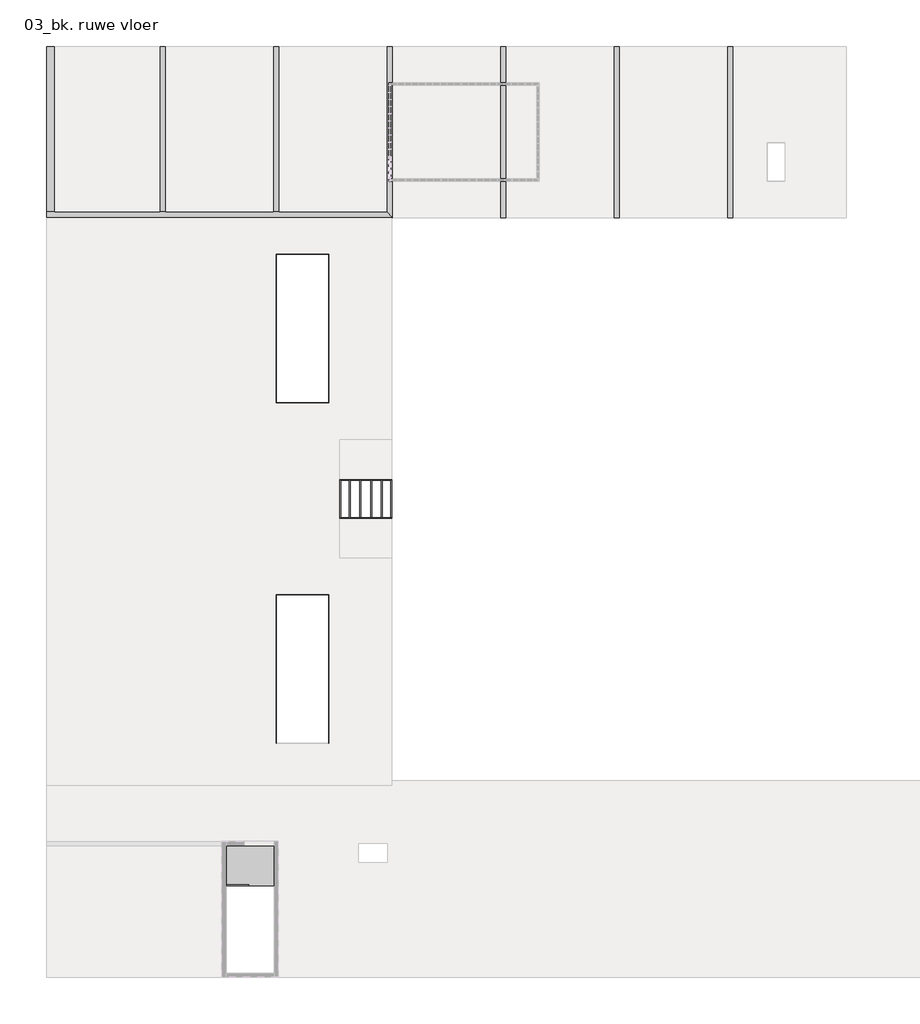
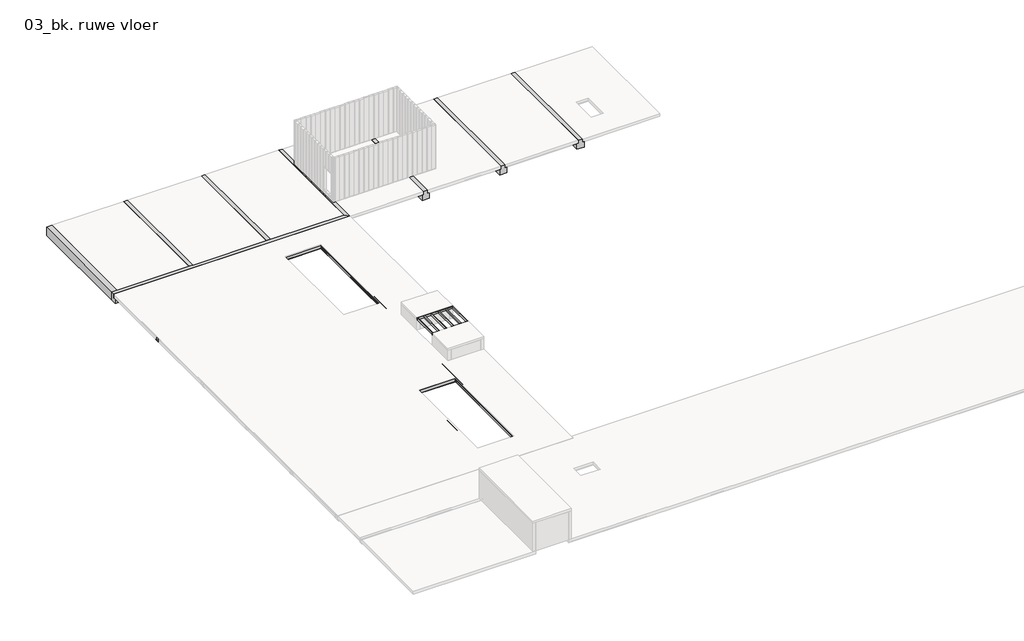
# One storey, part 9 of 9: 26 beams, 1 stair.
"""IFC4 building model written with IfcOpenShell, lengths in millimetres."""

import ifcopenshell
import ifcopenshell.guid

model = None  # the IFC model being written
_history = None  # IfcOwnerHistory: only IFC2X3 demands one
_inside = {}  # id of a spatial element -> (the spatial element, [elements in it])
_under = {}  # id of a project, library or spatial element -> (it, [spatial elements below it])
_declared = {}  # id of a project -> (the project, [libraries it declares])
_typed = {}  # id of a type object -> (the type object, [elements of that type])
_made_of = {}  # id of a material, layer set ... -> (it, [elements and type objects made of it])


def new_model(schema):
    """Start an empty IFC model of exactly this schema.

    Asked for "IFC4X3", IfcOpenShell would pick the latest addendum, in which some entities
    have other attributes; the version numbers below select the first issue.
    IFC2X3 requires an IfcOwnerHistory on every rooted entity: one is made here for all.
    """
    global model, _history
    if schema == "IFC4X3":
        model = ifcopenshell.file(schema_version=(4, 3, 0, 0))
    else:
        model = ifcopenshell.file(schema=schema)
    _inside.clear()
    _under.clear()
    _declared.clear()
    _typed.clear()
    _made_of.clear()
    _history = None
    if model.schema == "IFC2X3":
        org = make("IfcOrganization", Name="unknown")
        user = make(
            "IfcPersonAndOrganization",
            ThePerson=make("IfcPerson", FamilyName="unknown"),
            TheOrganization=org,
        )
        app = make(
            "IfcApplication",
            ApplicationDeveloper=org,
            Version="unknown",
            ApplicationFullName="unknown",
            ApplicationIdentifier="unknown",
        )
        _history = make(
            "IfcOwnerHistory",
            OwningUser=user,
            OwningApplication=app,
            ChangeAction="ADDED",
            CreationDate=0,
        )
    return model


def make(cls, **values):
    """One entity of the class cls with the attributes given. An attribute that is None is left unset."""
    return model.create_entity(
        cls, **{name: value for name, value in values.items() if value is not None}
    )


def rooted(cls, **values):
    """An entity with a GlobalId (a new one), such as an element, a storey or a relation."""
    return make(cls, GlobalId=ifcopenshell.guid.new(), OwnerHistory=_history, **values)


def si_unit(unit_type, name, prefix=None):
    """IfcSIUnit, for example si_unit("LENGTHUNIT", "METRE", prefix="MILLI")."""
    return make("IfcSIUnit", UnitType=unit_type, Prefix=prefix, Name=name)


def assignment(units):
    """IfcUnitAssignment: the units of a project."""
    return None if units is None else make("IfcUnitAssignment", Units=units)


def point(xyz):
    """IfcCartesianPoint."""
    return None if xyz is None else make("IfcCartesianPoint", Coordinates=xyz)


def direction(xyz):
    """IfcDirection."""
    return None if xyz is None else make("IfcDirection", DirectionRatios=xyz)


def frame(location, z_axis=None, x_axis=None):
    """IfcAxis2Placement3D, a coordinate frame: its origin and axes. An axis left out is left unset."""
    return make(
        "IfcAxis2Placement3D",
        Location=point(location),
        Axis=direction(z_axis),
        RefDirection=direction(x_axis),
    )


def frame_2d(location, x_axis=None):
    """IfcAxis2Placement2D, a coordinate frame in the plane: its origin and x axis."""
    return make(
        "IfcAxis2Placement2D", Location=point(location), RefDirection=direction(x_axis)
    )


def origin():
    """The frame at (0, 0, 0) with its axes left unset."""
    return frame((0.0, 0.0, 0.0))


def place(relative_to, where):
    """IfcLocalPlacement: puts the frame where relative to a parent placement (None: the world)."""
    return make(
        "IfcLocalPlacement", PlacementRelTo=relative_to, RelativePlacement=where
    )


def context(
    kind, dimensions, precision=None, world=None, true_north=None, identifier=None
):
    """IfcGeometricRepresentationContext, for example the 3D "Model" context."""
    return make(
        "IfcGeometricRepresentationContext",
        ContextIdentifier=identifier,
        ContextType=kind,
        CoordinateSpaceDimension=dimensions,
        Precision=precision,
        WorldCoordinateSystem=world,
        TrueNorth=true_north,
    )


def project(units=None, contexts=None):
    """IfcProject with its units and contexts."""
    return rooted(
        "IfcProject",
        Name="project",
        RepresentationContexts=contexts,
        UnitsInContext=assignment(units),
    )


def spatial(cls, under=None, at=None, **own):
    """A site, building, storey or space (cls), placed at a placement, below another one or the project."""
    s = rooted(cls, ObjectPlacement=at, **own)
    if under is not None:
        _under.setdefault(under.id(), (under, []))[1].append(s)
    return s


def polyline(points):
    """IfcPolyline through the points."""
    return make("IfcPolyline", Points=[point(p) for p in points])


def circle_curve(where, radius):
    """IfcCircle in the frame where."""
    return make("IfcCircle", Position=where, Radius=radius)


def trimmed(basis, trim1, trim2, sense, master):
    """IfcTrimmedCurve: the piece of a basis curve between two trims."""
    return make(
        "IfcTrimmedCurve",
        BasisCurve=basis,
        Trim1=trim1,
        Trim2=trim2,
        SenseAgreement=sense,
        MasterRepresentation=master,
    )


def segment(curve, same_sense, transition):
    """IfcCompositeCurveSegment."""
    return make(
        "IfcCompositeCurveSegment",
        Transition=transition,
        SameSense=same_sense,
        ParentCurve=curve,
    )


def composite_curve(segments, self_intersect=None):
    """IfcCompositeCurve: segments joined end to end."""
    return make("IfcCompositeCurve", Segments=segments, SelfIntersect=self_intersect)


def outline(outer, holes=None, kind="AREA"):
    """IfcArbitraryClosedProfileDef: a profile drawn as a closed curve; with holes, ...WithVoids."""
    if holes is None:
        return make("IfcArbitraryClosedProfileDef", ProfileType=kind, OuterCurve=outer)
    return make(
        "IfcArbitraryProfileDefWithVoids",
        ProfileType=kind,
        OuterCurve=outer,
        InnerCurves=holes,
    )


def extrude(swept, where, along, depth):
    """IfcExtrudedAreaSolid: the profile swept, set in the frame where, extruded along a direction by depth."""
    return make(
        "IfcExtrudedAreaSolid",
        SweptArea=swept,
        Position=where,
        ExtrudedDirection=direction(along),
        Depth=depth,
    )


def faces_of(points, faces, orient=None, outer=None):
    """IfcFace entities. A face is a list of loops; a loop is a list of indices into points, from 0.

    orient and outer hold one flag for each loop. By default every Orientation is true, the
    first loop of a face is its IfcFaceOuterBound and the others are IfcFaceBound.
    """
    made = []
    for i, loops in enumerate(faces):
        bounds = []
        for j, loop in enumerate(loops):
            is_outer = j == 0 if outer is None else outer[i][j]
            bounds.append(
                make(
                    "IfcFaceOuterBound" if is_outer else "IfcFaceBound",
                    Bound=make("IfcPolyLoop", Polygon=[points[k] for k in loop]),
                    Orientation=True if orient is None else orient[i][j],
                )
            )
        made.append(make("IfcFace", Bounds=bounds))
    return made


def faceted_brep(points, faces, orient=None, outer=None, voids=None):
    """IfcFacetedBrep: a solid bounded by flat faces; with voids (closed shells), ...WithVoids."""
    shared = [point(p) for p in points]
    hull = make("IfcClosedShell", CfsFaces=faces_of(shared, faces, orient, outer))
    if voids is None:
        return make("IfcFacetedBrep", Outer=hull)
    return make(
        "IfcFacetedBrepWithVoids",
        Outer=hull,
        Voids=[
            make(cls, CfsFaces=faces_of(shared, fs, o, b)) for cls, fs, o, b in voids
        ],
    )


def shape(context_of_items, identifier, shape_type, items):
    """IfcShapeRepresentation: the items that make up one representation, for example the "Body"."""
    return make(
        "IfcShapeRepresentation",
        ContextOfItems=context_of_items,
        RepresentationIdentifier=identifier,
        RepresentationType=shape_type,
        Items=items,
    )


def source(mapping_origin, context_of_items, identifier, shape_type, items):
    """IfcRepresentationMap: a shape defined once, which mapped items show again and again."""
    return make(
        "IfcRepresentationMap",
        MappingOrigin=mapping_origin,
        MappedRepresentation=shape(context_of_items, identifier, shape_type, items),
    )


def transform(
    local_origin,
    x_axis=None,
    y_axis=None,
    z_axis=None,
    scale=None,
    scale2=None,
    scale3=None,
    uniform=True,
):
    """IfcCartesianTransformationOperator3D, or its non-uniform kind. x_axis, y_axis, z_axis: its Axis1, 2, 3."""
    if uniform:
        return make(
            "IfcCartesianTransformationOperator3D",
            Axis1=direction(x_axis),
            Axis2=direction(y_axis),
            LocalOrigin=point(local_origin),
            Scale=scale,
            Axis3=direction(z_axis),
        )
    return make(
        "IfcCartesianTransformationOperator3DnonUniform",
        Axis1=direction(x_axis),
        Axis2=direction(y_axis),
        LocalOrigin=point(local_origin),
        Scale=scale,
        Axis3=direction(z_axis),
        Scale2=scale2,
        Scale3=scale3,
    )


def mapped(mapping_source, mapping_target):
    """IfcMappedItem: shows the shape of a source again, moved by a transform."""
    return make(
        "IfcMappedItem", MappingSource=mapping_source, MappingTarget=mapping_target
    )


def made_of(thing, what):
    """Note that an element or type object is made of a material, layer set ...; save() writes the relation."""
    if what is not None:
        _made_of.setdefault(what.id(), (what, []))[1].append(thing)
    return thing


def element(
    cls,
    number,
    at=None,
    inside=None,
    cuts=None,
    type_object=None,
    material=None,
    context=None,
    identifier="Body",
    shape_type=None,
    held_by="IfcProductDefinitionShape",
    body=None,
    shapes=None,
    **own,
):
    """One element of the class cls, such as IfcWall. Its Tag is "e" and its number.

    at: its placement. inside: the storey or other place that contains it. cuts: it is an
    opening in that element (IfcRelVoidsElement). A single representation is given by context,
    identifier, shape_type and body (its items); several are given by shapes. held_by: the class
    of the entity that holds the representations. save() writes the other relations.
    """
    e = rooted(cls, Tag="e%d" % number, ObjectPlacement=at, **own)
    if body is not None:
        shapes = [shape(context, identifier, shape_type, body)]
    if shapes is not None:
        e.Representation = make(held_by, Representations=shapes)
    if inside is not None:
        _inside.setdefault(inside.id(), (inside, []))[1].append(e)
    if cuts is not None:
        rooted(
            "IfcRelVoidsElement", RelatingBuildingElement=cuts, RelatedOpeningElement=e
        )
    if type_object is not None:
        _typed.setdefault(type_object.id(), (type_object, []))[1].append(e)
    return made_of(e, material)


def aggregate(whole, parts):
    """IfcRelAggregates: a whole, such as a stair, and the parts it consists of."""
    return rooted("IfcRelAggregates", RelatingObject=whole, RelatedObjects=parts)


def save(model, path):
    """Write the relations noted so far, then the file.

    IfcRelAggregates (storeys below a building ...), IfcRelContainedInSpatialStructure (elements
    in a storey), IfcRelDefinesByType, IfcRelAssociatesMaterial and IfcRelDeclares: one each for
    every whole, place, type object, material and project.
    """
    for whole, parts in _under.values():
        aggregate(whole, parts)
    for where, things in _inside.values():
        rooted(
            "IfcRelContainedInSpatialStructure",
            RelatedElements=things,
            RelatingStructure=where,
        )
    for kind, things in _typed.values():
        rooted("IfcRelDefinesByType", RelatedObjects=things, RelatingType=kind)
    for what, things in _made_of.values():
        rooted("IfcRelAssociatesMaterial", RelatedObjects=things, RelatingMaterial=what)
    for by, libraries in _declared.values():
        rooted("IfcRelDeclares", RelatingContext=by, RelatedDefinitions=libraries)
    model.write(path)


def beam_736acf17(model_context):
    return source(origin(), model_context, "Body", "SweptSolid", [
        extrude(outline(polyline([(143.5, 280.0), (143.5, 0.0), (263.5, 0.0), (263.5, -20.0), (-286.5, -20.0), (-286.5, 0.0), (-166.5, 0.0), (-166.5, 280.0), (143.5, 280.0)]), holes=[polyline([(133.5, 0.0), (133.5, 250.0), (-156.5, 250.0), (-156.5, 0.0), (133.5, 0.0)])]), frame((-6445.0, 0.0, 0.0), z_axis=(1.0, 0.0, 0.0), x_axis=(0.0, 1.0, 0.0)), (0.0, 0.0, 1.0), 12890.0),
    ])


def beam_bc03ea60(model_context):
    return source(origin(), model_context, "Body", "SweptSolid", [
        extrude(outline(polyline([(-139.5, 280.0), (162.5, 280.0), (162.5, 0.0), (172.5, 0.0), (172.5, -15.0), (-277.5, -15.0), (-277.5, 0.0), (-139.5, 0.0), (-139.5, 280.0)]), holes=[polyline([(-133.5, 0.0), (156.5, 0.0), (156.5, 250.0), (-133.5, 250.0), (-133.5, 0.0)])]), frame((-1499.9999994, 0.0, 0.0), z_axis=(1.0, 0.0, 0.0), x_axis=(0.0, 1.0, 0.0)), (0.0, 0.0, 1.0), 2999.9999988),
    ])


def beam_09e22bfa(model_context):
    return source(origin(), model_context, "Body", "SweptSolid", [
        extrude(outline(polyline([(143.5, 280.0), (143.5, 0.0), (263.5, 0.0), (263.5, -20.0), (-286.5, -20.0), (-286.5, 0.0), (-166.5, 0.0), (-166.5, 280.0), (143.5, 280.0)]), holes=[polyline([(133.5, 0.0), (133.5, 250.0), (-156.5, 250.0), (-156.5, 0.0), (133.5, 0.0)])]), frame((-1682.5, 0.0, 0.0), z_axis=(1.0, 0.0, 0.0), x_axis=(0.0, 1.0, 0.0)), (0.0, 0.0, 1.0), 3365.0),
    ])


def beam_7c9e214b(model_context):
    return source(origin(), model_context, "Body", "SweptSolid", [
        extrude(outline(polyline([(139.5, 280.0), (139.5, 0.0), (277.5, 0.0), (277.5, -15.0), (-172.5, -15.0), (-172.5, 0.0), (-162.5, 0.0), (-162.5, 280.0), (139.5, 280.0)]), holes=[polyline([(133.5, 0.0), (133.5, 250.0), (-156.5, 250.0), (-156.5, 0.0), (133.5, 0.0)])]), frame((-1499.9999994, 0.0, 0.0), z_axis=(1.0, 0.0, 0.0), x_axis=(0.0, 1.0, 0.0)), (0.0, 0.0, 1.0), 2999.9999988),
    ])


def beam_87fc56b5(model_context):
    return source(origin(), model_context, "Body", "SweptSolid", [
        extrude(outline(polyline([(143.5, 280.0), (143.5, 0.0), (263.5, 0.0), (263.5, -20.0), (-286.5, -20.0), (-286.5, 0.0), (-166.5, 0.0), (-166.5, 280.0), (143.5, 280.0)]), holes=[polyline([(133.5, 0.0), (133.5, 250.0), (-156.5, 250.0), (-156.5, 0.0), (133.5, 0.0)])]), frame((-1812.5, 0.0, 0.0), z_axis=(1.0, 0.0, 0.0), x_axis=(0.0, 1.0, 0.0)), (0.0, 0.0, 1.0), 3365.0),
    ])


def beam_01d7d33a(model_context):
    return source(origin(), model_context, "Body", "SweptSolid", [
        extrude(outline(composite_curve([segment(polyline([(130.0, 112.5), (29.0, 112.5)]), True, "CONTINUOUS"), segment(trimmed(circle_curve(frame_2d((29.0, 88.5)), 24.0), [point((29.0, 112.5))], [point((5.0, 88.5))], True, "CARTESIAN"), True, "CONTINUOUS"), segment(polyline([(5.0, 88.5), (5.0, -88.5)]), True, "CONTINUOUS"), segment(trimmed(circle_curve(frame_2d((29.0, -88.5)), 24.0), [point((5.0, -88.5))], [point((29.0, -112.5))], True, "CARTESIAN"), True, "CONTINUOUS"), segment(polyline([(29.0, -112.5), (130.0, -112.5), (130.0, -130.0), (-130.0, -130.0), (-130.0, -112.5), (-29.0, -112.5)]), True, "CONTINUOUS"), segment(trimmed(circle_curve(frame_2d((-29.0, -88.5)), 24.0), [point((-29.0, -112.5))], [point((-5.0, -88.5))], True, "CARTESIAN"), True, "CONTINUOUS"), segment(polyline([(-5.0, -88.5), (-5.0, 88.5)]), True, "CONTINUOUS"), segment(trimmed(circle_curve(frame_2d((-29.0, 88.5)), 24.0), [point((-5.0, 88.5))], [point((-29.0, 112.5))], True, "CARTESIAN"), True, "CONTINUOUS"), segment(polyline([(-29.0, 112.5), (-130.0, 112.5), (-130.0, 130.0), (130.0, 130.0), (130.0, 112.5)]), True, "CONTINUOUS")], self_intersect=False)), frame((-6349.0, 0.0, 0.0), z_axis=(1.0, 0.0, 0.0), x_axis=(0.0, 1.0, 0.0)), (0.0, 0.0, 1.0), 12698.0),
    ])


def beam_3eaeb734(model_context):
    return source(origin(), model_context, "Body", "SweptSolid", [
        extrude(outline(composite_curve([segment(polyline([(-130.0, 112.5), (-130.0, 130.0), (130.0, 130.0), (130.0, 112.5), (29.0, 112.5)]), True, "CONTINUOUS"), segment(trimmed(circle_curve(frame_2d((29.0, 88.5)), 24.0), [point((29.0, 112.5))], [point((5.0, 88.5))], True, "CARTESIAN"), True, "CONTINUOUS"), segment(polyline([(5.0, 88.5), (5.0, -88.5)]), True, "CONTINUOUS"), segment(trimmed(circle_curve(frame_2d((29.0, -88.5)), 24.0), [point((5.0, -88.5))], [point((29.0, -112.5))], True, "CARTESIAN"), True, "CONTINUOUS"), segment(polyline([(29.0, -112.5), (130.0, -112.5), (130.0, -130.0), (-130.0, -130.0), (-130.0, -112.5), (-29.0, -112.5)]), True, "CONTINUOUS"), segment(trimmed(circle_curve(frame_2d((-29.0, -88.5)), 24.0), [point((-29.0, -112.5))], [point((-5.0, -88.5))], True, "CARTESIAN"), True, "CONTINUOUS"), segment(polyline([(-5.0, -88.5), (-5.0, 88.5)]), True, "CONTINUOUS"), segment(trimmed(circle_curve(frame_2d((-29.0, 88.5)), 24.0), [point((-5.0, 88.5))], [point((-29.0, 112.5))], True, "CARTESIAN"), True, "CONTINUOUS"), segment(polyline([(-29.0, 112.5), (-130.0, 112.5)]), True, "CONTINUOUS")], self_intersect=False)), frame((-6349.0, 0.0, 0.0), z_axis=(1.0, 0.0, 0.0), x_axis=(0.0, 1.0, 0.0)), (0.0, 0.0, 1.0), 12698.0),
    ])


def beam_0ced8335(model_context):
    return source(origin(), model_context, "Body", "SweptSolid", [
        extrude(outline(composite_curve([segment(polyline([(130.0, 112.5), (29.0, 112.5)]), True, "CONTINUOUS"), segment(trimmed(circle_curve(frame_2d((29.0, 88.5)), 24.0), [point((29.0, 112.5))], [point((5.0, 88.5))], True, "CARTESIAN"), True, "CONTINUOUS"), segment(polyline([(5.0, 88.5), (5.0, -88.5)]), True, "CONTINUOUS"), segment(trimmed(circle_curve(frame_2d((29.0, -88.5)), 24.0), [point((5.0, -88.5))], [point((29.0, -112.5))], True, "CARTESIAN"), True, "CONTINUOUS"), segment(polyline([(29.0, -112.5), (130.0, -112.5), (130.0, -130.0), (-130.0, -130.0), (-130.0, -112.5), (-29.0, -112.5)]), True, "CONTINUOUS"), segment(trimmed(circle_curve(frame_2d((-29.0, -88.5)), 24.0), [point((-29.0, -112.5))], [point((-5.0, -88.5))], True, "CARTESIAN"), True, "CONTINUOUS"), segment(polyline([(-5.0, -88.5), (-5.0, 88.5)]), True, "CONTINUOUS"), segment(trimmed(circle_curve(frame_2d((-29.0, 88.5)), 24.0), [point((-5.0, 88.5))], [point((-29.0, 112.5))], True, "CARTESIAN"), True, "CONTINUOUS"), segment(polyline([(-29.0, 112.5), (-130.0, 112.5), (-130.0, 130.0), (130.0, 130.0), (130.0, 112.5)]), True, "CONTINUOUS")], self_intersect=False)), frame((-6318.75, 0.0, 0.0), z_axis=(1.0, 0.0, 0.0), x_axis=(0.0, 1.0, 0.0)), (0.0, 0.0, 1.0), 12637.5),
    ])


def beam_f33d2ea4(model_context):
    return source(origin(), model_context, "Body", "SweptSolid", [
        extrude(outline(composite_curve([segment(polyline([(-130.0, 112.5), (-130.0, 130.0), (130.0, 130.0), (130.0, 112.5), (29.0, 112.5)]), True, "CONTINUOUS"), segment(trimmed(circle_curve(frame_2d((29.0, 88.5)), 24.0), [point((29.0, 112.5))], [point((5.0, 88.5))], True, "CARTESIAN"), True, "CONTINUOUS"), segment(polyline([(5.0, 88.5), (5.0, -88.5)]), True, "CONTINUOUS"), segment(trimmed(circle_curve(frame_2d((29.0, -88.5)), 24.0), [point((5.0, -88.5))], [point((29.0, -112.5))], True, "CARTESIAN"), True, "CONTINUOUS"), segment(polyline([(29.0, -112.5), (130.0, -112.5), (130.0, -130.0), (-130.0, -130.0), (-130.0, -112.5), (-29.0, -112.5)]), True, "CONTINUOUS"), segment(trimmed(circle_curve(frame_2d((-29.0, -88.5)), 24.0), [point((-29.0, -112.5))], [point((-5.0, -88.5))], True, "CARTESIAN"), True, "CONTINUOUS"), segment(polyline([(-5.0, -88.5), (-5.0, 88.5)]), True, "CONTINUOUS"), segment(trimmed(circle_curve(frame_2d((-29.0, 88.5)), 24.0), [point((-5.0, 88.5))], [point((-29.0, 112.5))], True, "CARTESIAN"), True, "CONTINUOUS"), segment(polyline([(-29.0, 112.5), (-130.0, 112.5)]), True, "CONTINUOUS")], self_intersect=False)), frame((-6318.75, 0.0, 0.0), z_axis=(1.0, 0.0, 0.0), x_axis=(0.0, 1.0, 0.0)), (0.0, 0.0, 1.0), 12637.5),
    ])


def beam_e7c6e874(model_context):
    return source(origin(), model_context, "Body", "SweptSolid", [
        extrude(outline(polyline([(-1067.0, -29.0), (-1067.0, 29.0), (1067.0, 29.0), (1067.0, -29.0), (-1067.0, -29.0)])), frame((0.0, 0.0, -78.0), z_axis=(0.0, 0.0, 1.0), x_axis=(1.0, 0.0, 0.0)), (0.0, 0.0, 1.0), 156.0),
    ])


def stair_f79be4d1(model_context):
    return source(origin(), model_context, "Body", "Brep", [
        faceted_brep([(1365.0, -2300.0, 0.0), (1365.0, -2300.0, -60.0), (1365.0, 0.0, -60.0), (1365.0, 0.0, 0.0), (-55.0, -2300.0, 0.0), (-55.0, -2190.0, 0.0), (-55.0, -2190.0, -110.0), (-55.0, -2300.0, -110.0), (-1365.0, 0.0, 0.0), (-1365.0, 0.0, -60.0), (-1365.0, -2190.0, -60.0), (-1365.0, -2190.0, 0.0), (-1335.0, -2300.0, -110.0), (-1335.0, -2300.0, -200.0), (-1210.0, -2300.0, -200.0), (-1210.0, -2300.0, -220.0), (1210.0, -2300.0, -220.0), (1210.0, -2300.0, -200.0), (1335.0, -2300.0, -200.0), (1335.0, -2300.0, -60.0), (-1335.0, -2190.0, -110.0), (-1335.0, -2190.0, -60.0), (1335.0, 0.0, -60.0), (1335.0, 0.0, -200.0), (1210.0, 0.0, -200.0), (1210.0, 0.0, -220.0), (-1210.0, 0.0, -220.0), (-1210.0, 0.0, -200.0), (-1335.0, 0.0, -200.0), (-1335.0, 0.0, -60.0)], [[[0, 1, 2, 3]], [[4, 5, 6, 7]], [[8, 9, 10, 11]], [[12, 13, 14, 15, 16, 17, 18, 19, 1, 0, 4, 7]], [[7, 6, 20, 12]], [[11, 10, 21, 20, 6, 5]], [[11, 5, 4, 0, 3, 8]], [[8, 3, 2, 22, 23, 24, 25, 26, 27, 28, 29, 9]], [[26, 25, 16, 15]], [[21, 10, 9, 29]], [[13, 12, 20, 21, 29, 28]], [[28, 27, 14, 13]], [[27, 26, 15, 14]], [[22, 2, 1, 19]], [[19, 18, 23, 22]], [[18, 17, 24, 23]], [[17, 16, 25, 24]]]),
    ])


model = new_model("IFC4")

# Units and contexts
model_context = context("Model", 3, world=origin())
ifc_project = project(units=[si_unit("LENGTHUNIT", "METRE", prefix="MILLI")], contexts=[model_context])

# Site, building, storey
site = spatial("IfcSite", under=ifc_project)
building = spatial("IfcBuilding", under=site)
storey = spatial("IfcBuildingStorey", under=building, Name="03_bk. ruwe vloer", Elevation=11330.0)

# Beams
placement = place(None, origin())
element("IfcBeam", 1, ObjectType="NLRS_28_SF_LIB_balk dubbele sponning beton prefab-CWV-MMBC-SRP_gen_rsf : balk beton prefab_gen__bxh 600x750 dubbele inkassing bxh 120x260", at=placement, inside=storey, context=model_context, shape_type="Brep", body=[
    faceted_brep([(32680.0, 43350.0, 11330.0), (32320.0, 43350.0, 11330.0), (32320.0, 43350.0, 11070.0), (32200.0, 43350.0, 11070.0), (32200.0, 43350.0, 10580.0), (32800.0, 43350.0, 10580.0), (32800.0, 43350.0, 11070.0), (32680.0, 43350.0, 11070.0), (32680.0, 53150.0, 11330.0), (32680.0, 53150.0, 11070.0), (32800.0, 53150.0, 11070.0), (32800.0, 53150.0, 10580.0), (32200.0, 53150.0, 10580.0), (32200.0, 53150.0, 11070.0), (32320.0, 53150.0, 11070.0), (32320.0, 53150.0, 11330.0), (32200.0, 53140.0, 11070.0), (32200.0, 43360.0, 11070.0), (32800.0, 53140.0, 11070.0), (32800.0, 43360.0, 11070.0)], [[[0, 1, 2, 3, 4, 5, 6, 7]], [[8, 9, 10, 11, 12, 13, 14, 15]], [[1, 0, 8, 15]], [[2, 1, 15, 14]], [[3, 2, 14, 13, 16, 17]], [[4, 3, 17, 16, 13, 12]], [[5, 4, 12, 11]], [[6, 5, 11, 10, 18, 19]], [[7, 6, 19, 18, 10, 9]], [[0, 7, 9, 8]]]),
])
element("IfcBeam", 2, ObjectType="NLRS_28_SF_LIB_balk dubbele sponning beton prefab-CWV-MMBC-SRP_gen_rsf : balk beton prefab_gen__bxh 600x750 dubbele inkassing bxh 120x260", at=placement, inside=storey, context=model_context, shape_type="Brep", body=[
    faceted_brep([(39180.0, 43350.0, 11330.0), (38820.0, 43350.0, 11330.0), (38820.0, 43350.0, 11070.0), (38700.0, 43350.0, 11070.0), (38700.0, 43350.0, 10580.0), (39300.0, 43350.0, 10580.0), (39300.0, 43350.0, 11070.0), (39180.0, 43350.0, 11070.0), (39180.0, 53150.0, 11330.0), (39180.0, 53150.0, 11070.0), (39300.0, 53150.0, 11070.0), (39300.0, 53150.0, 10580.0), (38700.0, 53150.0, 10580.0), (38700.0, 53150.0, 11070.0), (38820.0, 53150.0, 11070.0), (38820.0, 53150.0, 11330.0), (38700.0, 53140.0, 11070.0), (38700.0, 43360.0, 11070.0), (39300.0, 53140.0, 11070.0), (39300.0, 43360.0, 11070.0)], [[[0, 1, 2, 3, 4, 5, 6, 7]], [[8, 9, 10, 11, 12, 13, 14, 15]], [[1, 0, 8, 15]], [[2, 1, 15, 14]], [[3, 2, 14, 13, 16, 17]], [[4, 3, 17, 16, 13, 12]], [[5, 4, 12, 11]], [[6, 5, 11, 10, 18, 19]], [[7, 6, 19, 18, 10, 9]], [[0, 7, 9, 8]]]),
])
element("IfcBeam", 3, ObjectType="NLRS_28_SF_LIB_balk dubbele sponning beton prefab-CWV-MMBC-SRP_gen_rsf : balk beton prefab_gen__bxh 600x750 dubbele inkassing bxh 120x260", at=placement, inside=storey, context=model_context, shape_type="Brep", body=[
    faceted_brep([(45680.0, 43350.0, 11330.0), (45320.0, 43350.0, 11330.0), (45320.0, 43350.0, 11070.0), (45200.0, 43350.0, 11070.0), (45200.0, 43350.0, 10580.0), (45800.0, 43350.0, 10580.0), (45800.0, 43350.0, 11070.0), (45680.0, 43350.0, 11070.0), (45680.0, 53150.0, 11330.0), (45680.0, 53150.0, 11070.0), (45800.0, 53150.0, 11070.0), (45800.0, 53150.0, 10580.0), (45200.0, 53150.0, 10580.0), (45200.0, 53150.0, 11070.0), (45320.0, 53150.0, 11070.0), (45320.0, 53150.0, 11330.0), (45200.0, 53140.0, 11070.0), (45200.0, 43360.0, 11070.0), (45800.0, 53140.0, 11070.0), (45800.0, 43360.0, 11070.0)], [[[0, 1, 2, 3, 4, 5, 6, 7]], [[8, 9, 10, 11, 12, 13, 14, 15]], [[1, 0, 8, 15]], [[2, 1, 15, 14]], [[3, 2, 14, 13, 16, 17]], [[4, 3, 17, 16, 13, 12]], [[5, 4, 12, 11]], [[6, 5, 11, 10, 18, 19]], [[7, 6, 19, 18, 10, 9]], [[0, 7, 9, 8]]]),
])
element("IfcBeam", 4, ObjectType="NLRS_28_SF_LIB_balk dubbele sponning beton prefab-CWV-MMBC-SRP_gen_rsf : balk beton prefab_gen__bxh 600x750 dubbele inkassing bxh 120x260", at=placement, inside=storey, context=model_context, shape_type="Brep", body=[
    faceted_brep([(26180.0, 53150.0, 11330.0), (26180.0, 53150.0, 11070.0), (26300.0, 53150.0, 11070.0), (26300.0, 53150.0, 10580.0), (25700.0, 53150.0, 10580.0), (25700.0, 53150.0, 11070.0), (25820.0, 53150.0, 11070.0), (25820.0, 53150.0, 11330.0), (25820.0, 43680.0, 11330.0), (26150.0, 43350.0, 11330.0), (26180.0, 43350.0, 11330.0), (25820.0, 43680.0, 11070.0), (25700.0, 53140.0, 11070.0), (25700.0, 43800.0, 11070.0), (25725.0, 43775.0, 11070.0), (25700.0, 43800.0, 10580.0), (26300.0, 43350.0, 10580.0), (26150.0, 43350.0, 10580.0), (26300.0, 53140.0, 11070.0), (26300.0, 43360.0, 11070.0), (26300.0, 43350.0, 11070.0), (26180.0, 43350.0, 11070.0)], [[[0, 1, 2, 3, 4, 5, 6, 7]], [[0, 7, 8, 9, 10]], [[7, 6, 11, 8]], [[6, 5, 12, 13, 14, 11]], [[5, 4, 15, 13, 12]], [[4, 3, 16, 17, 15]], [[3, 2, 18, 19, 20, 16]], [[2, 1, 21, 20, 19, 18]], [[1, 0, 10, 21]], [[8, 11, 14, 13, 15, 17, 9]], [[17, 16, 20, 21, 10, 9]]]),
])
element("IfcBeam", 5, ObjectType="NLRS_28_SF_LIB_balk dubbele sponning beton prefab-CWV-MMBC-SRP_gen_rsf : balk beton prefab_gen__bxh 600x750 dubbele inkassing bxh 120x260", at=placement, inside=storey, context=model_context, shape_type="Brep", body=[
    faceted_brep([(19680.0, 53150.0, 11330.0), (19680.0, 53150.0, 11070.0), (19800.0, 53150.0, 11070.0), (19800.0, 53150.0, 10580.0), (19200.0, 53150.0, 10580.0), (19200.0, 53150.0, 11070.0), (19320.0, 53150.0, 11070.0), (19320.0, 53150.0, 11330.0), (19320.0, 43680.0, 11330.0), (19680.0, 43680.0, 11330.0), (19320.0, 43800.0, 11070.0), (19320.0, 43680.0, 11070.0), (19200.0, 53140.0, 11070.0), (19200.0, 43800.0, 11070.0), (19225.0, 43800.0, 11070.0), (19200.0, 43800.0, 10580.0), (19800.0, 43800.0, 10580.0), (19800.0, 53140.0, 11070.0), (19800.0, 43800.0, 11070.0), (19680.0, 43800.0, 11070.0), (19775.0, 43800.0, 11070.0), (19680.0, 43680.0, 11070.0)], [[[0, 1, 2, 3, 4, 5, 6, 7]], [[0, 7, 8, 9]], [[7, 6, 10, 11, 8]], [[6, 5, 12, 13, 14, 10]], [[5, 4, 15, 13, 12]], [[4, 3, 16, 15]], [[3, 2, 17, 18, 16]], [[2, 1, 19, 20, 18, 17]], [[1, 0, 9, 21, 19]], [[19, 10, 14, 13, 15, 16, 18, 20]], [[21, 11, 10, 19]], [[11, 21, 9, 8]]]),
])
element("IfcBeam", 6, ObjectType="NLRS_28_SF_LIB_balk dubbele sponning beton prefab-CWV-MMBC-SRP_gen_rsf : balk beton prefab_gen__bxh 600x750 dubbele inkassing bxh 120x260", at=placement, inside=storey, context=model_context, shape_type="Brep", body=[
    faceted_brep([(13180.0, 53150.0, 11330.0), (13180.0, 53150.0, 11070.0), (13300.0, 53150.0, 11070.0), (13300.0, 53150.0, 10580.0), (12700.0, 53150.0, 10580.0), (12700.0, 53150.0, 11070.0), (12820.0, 53150.0, 11070.0), (12820.0, 53150.0, 11330.0), (12820.0, 43680.0, 11330.0), (13180.0, 43680.0, 11330.0), (12820.0, 43800.0, 11070.0), (12820.0, 43680.0, 11070.0), (12700.0, 53140.0, 11070.0), (12700.0, 43800.0, 11070.0), (12700.0, 43800.0, 10580.0), (13300.0, 43800.0, 10580.0), (13300.0, 53140.0, 11070.0), (13300.0, 43800.0, 11070.0), (13180.0, 43800.0, 11070.0), (13180.0, 43680.0, 11070.0)], [[[0, 1, 2, 3, 4, 5, 6, 7]], [[0, 7, 8, 9]], [[7, 6, 10, 11, 8]], [[6, 5, 12, 13, 10]], [[5, 4, 14, 13, 12]], [[4, 3, 15, 14]], [[3, 2, 16, 17, 15]], [[2, 1, 18, 17, 16]], [[1, 0, 9, 19, 18]], [[18, 10, 13, 14, 15, 17]], [[19, 11, 10, 18]], [[11, 19, 9, 8]]]),
])
element("IfcBeam", 7, ObjectType="NLRS_28_SF_LIB_balk enkele sponning beton prefab-CWV-MMBC-SRP_gen_rsf : balk beton prefab_gen__bxh 600x750 met inkassing bxh120x260", at=placement, inside=storey, context=model_context, shape_type="Brep", body=[
    faceted_brep([(6350.0, 43680.0, 11330.0), (6350.0, 43680.0, 10580.0), (6950.0, 43680.0, 10580.0), (6950.0, 43680.0, 11070.0), (6830.0, 43680.0, 11070.0), (6830.0, 43680.0, 11330.0), (6350.0, 53150.0, 11330.0), (6830.0, 53150.0, 11330.0), (6830.0, 53150.0, 11070.0), (6950.0, 53150.0, 11070.0), (6950.0, 53150.0, 10580.0), (6350.0, 53150.0, 10580.0), (6950.0, 43775.0, 11070.0), (6950.0, 43800.0, 11070.0), (6950.0, 53140.0, 11070.0), (6950.0, 43800.0, 10580.0)], [[[0, 1, 2, 3, 4, 5]], [[6, 7, 8, 9, 10, 11]], [[0, 5, 7, 6]], [[5, 4, 8, 7]], [[4, 3, 12, 13, 14, 9, 8]], [[3, 2, 15, 10, 9, 14, 13, 12]], [[2, 1, 11, 10, 15]], [[1, 0, 6, 11]]]),
])
element("IfcBeam", 8, ObjectType="NLRS_28_SF_LIB_balk dubbele sponning beton prefab-CWV-MMBC-SRP_gen_rsf : balk beton prefab_gen__bxh 600x750 dubbele inkassing bxh 120x260 en 150x330", at=placement, inside=storey, context=model_context, shape_type="Brep", body=[
    faceted_brep([(6350.0, 43350.0, 11330.0), (6350.0, 43680.0, 11330.0), (6350.0, 43680.0, 10580.0), (6350.0, 43200.0, 10580.0), (6350.0, 43200.0, 11000.0), (6350.0, 43330.0, 11000.0), (6350.0, 43350.0, 11000.0), (6350.0, 43350.0, 11260.0), (26125.0, 43350.0, 11330.0), (26150.0, 43350.0, 11330.0), (25820.0, 43680.0, 11330.0), (19680.0, 43680.0, 11330.0), (19320.0, 43680.0, 11330.0), (13180.0, 43680.0, 11330.0), (12820.0, 43680.0, 11330.0), (6830.0, 43680.0, 11330.0), (26125.0, 43350.0, 11000.0), (26125.0, 43350.0, 10580.0), (26150.0, 43350.0, 10580.0), (19240.0, 43200.0, 11000.0), (19500.0, 43200.0, 11000.0), (22500.0, 43200.0, 11000.0), (22760.0, 43200.0, 11000.0), (26125.0, 43200.0, 11000.0), (26125.0, 43330.0, 11000.0), (26125.0, 43200.0, 10580.0), (25700.0, 43800.0, 10580.0), (6950.0, 43680.0, 10580.0), (6950.0, 43800.0, 10580.0), (12700.0, 43800.0, 10580.0), (13300.0, 43800.0, 10580.0), (19200.0, 43800.0, 10580.0), (19800.0, 43800.0, 10580.0), (25700.0, 43800.0, 11070.0), (6950.0, 43800.0, 11070.0), (12700.0, 43800.0, 11070.0), (12725.0, 43800.0, 11070.0), (12820.0, 43800.0, 11070.0), (13180.0, 43800.0, 11070.0), (13275.0, 43800.0, 11070.0), (13300.0, 43800.0, 11070.0), (19200.0, 43800.0, 11070.0), (19225.0, 43800.0, 11070.0), (19320.0, 43800.0, 11070.0), (19680.0, 43800.0, 11070.0), (19775.0, 43800.0, 11070.0), (19800.0, 43800.0, 11070.0), (25820.0, 43680.0, 11070.0), (25725.0, 43775.0, 11070.0), (6950.0, 43775.0, 11070.0), (6950.0, 43680.0, 11070.0), (12820.0, 43680.0, 11070.0), (13180.0, 43680.0, 11070.0), (19320.0, 43680.0, 11070.0), (19680.0, 43680.0, 11070.0)], [[[0, 1, 2, 3, 4, 5, 6, 7]], [[1, 0, 8, 9, 10, 11, 12, 13, 14, 15]], [[6, 16, 17, 18, 9, 8, 0, 7]], [[16, 6, 5, 4, 19, 20, 21, 22, 23, 24]], [[4, 3, 25, 23, 22, 21, 20, 19]], [[26, 18, 17, 25, 3, 2, 27, 28, 29, 30, 31, 32]], [[33, 26, 32, 31, 30, 29, 28, 34, 35, 36, 37, 38, 39, 40, 41, 42, 43, 44, 45, 46]], [[47, 48, 33, 46, 45, 44, 43, 42, 41, 40, 39, 38, 37, 36, 35, 34, 49, 50, 51, 52, 53, 54]], [[10, 47, 54, 53, 52, 51, 50, 27, 2, 1, 15, 14, 13, 12, 11]], [[10, 9, 18, 26, 33, 48, 47]], [[34, 28, 27, 50, 49]], [[17, 16, 24, 23, 25]]]),
])
element("IfcBeam", 9, ObjectType="NLRS_28_SF_LIB_houten balk-MMBW-SRP_gen_rsf : houten balk_gen__bxh 58x156", at=placement, inside=storey, context=model_context, shape_type="SweptSolid", body=[
    extrude(outline(polyline([(26125.0, 26183.0), (26067.0, 26183.0), (26067.0, 28317.0), (26125.0, 28317.0), (26125.0, 26183.0)])), frame((0.0, 0.0, 12276.0), z_axis=(0.0, 0.0, 1.0), x_axis=(1.0, 0.0, 0.0)), (0.0, 0.0, 1.0), 156.0),
])
element("IfcBeam", 10, ObjectType="NLRS_28_SF_LIB_houten balk-MMBW-SRP_gen_rsf : houten balk_gen__bxh 58x156", at=placement, inside=storey, context=model_context, shape_type="SweptSolid", body=[
    extrude(outline(polyline([(23183.0, 26183.0), (23125.0, 26183.0), (23125.0, 28317.0), (23183.0, 28317.0), (23183.0, 26183.0)])), frame((0.0, 0.0, 12276.0), z_axis=(0.0, 0.0, 1.0), x_axis=(1.0, 0.0, 0.0)), (0.0, 0.0, 1.0), 156.0),
])
element("IfcBeam", 11, ObjectType="NLRS_28_SF_LIB_houten balk-MMBW-SRP_gen_rsf : houten balk_gen__bxh 58x156", at=placement, inside=storey, context=model_context, shape_type="SweptSolid", body=[
    extrude(outline(polyline([(23125.0, 28317.0), (23125.0, 28375.0), (26125.0, 28375.0), (26125.0, 28317.0), (23125.0, 28317.0)])), frame((0.0, 0.0, 12276.0), z_axis=(0.0, 0.0, 1.0), x_axis=(1.0, 0.0, 0.0)), (0.0, 0.0, 1.0), 156.0),
])
element("IfcBeam", 12, ObjectType="NLRS_28_SF_LIB_houten balk-MMBW-SRP_gen_rsf : houten balk_gen__bxh 58x156", at=placement, inside=storey, context=model_context, shape_type="SweptSolid", body=[
    extrude(outline(polyline([(23125.0, 26183.0), (26125.0, 26183.0), (26125.0, 26125.0), (23125.0, 26125.0), (23125.0, 26183.0)])), frame((0.0, 0.0, 12276.0), z_axis=(0.0, 0.0, 1.0), x_axis=(1.0, 0.0, 0.0)), (0.0, 0.0, 1.0), 156.0),
])
beam_shape = beam_736acf17(model_context)
element("IfcBeam", 13, ObjectType="NLRS_28_SF_LIB_stalen ligger THQ-AV-CWV-MMBS-SRP_gen_rsf : stalen ligger_gen__THQ_280x10-290x30-550x20", at=placement, inside=storey, context=model_context, shape_type="MappedRepresentation", body=[
    mapped(beam_shape, transform((12795.0, 36988.5, 11000.0), x_axis=(-1.0, 0.0, 0.0), y_axis=(0.0, -1.0, 0.0), z_axis=(0.0, 0.0, 1.0))),
])
beam_2_shape = beam_bc03ea60(model_context)
element("IfcBeam", 14, ObjectType="NLRS_28_SF_LIB_stalen ligger THQ-AV-CWV-MMBS-SRP_gen_rsf : stalen ligger_gen__PET 280x6-290x30-450x15", at=placement, inside=storey, context=model_context, shape_type="MappedRepresentation", body=[
    mapped(beam_2_shape, transform((21000.0, 21922.5, 11000.0), x_axis=(-1.0, 0.0, 0.0), y_axis=(0.0, -1.0, 0.0), z_axis=(0.0, 0.0, 1.0))),
])
element("IfcBeam", 15, ObjectType="NLRS_28_SF_LIB_stalen ligger THQ-AV-CWV-MMBS-SRP_gen_rsf : stalen ligger_gen__PET 280x6-290x30-450x15", at=placement, inside=storey, context=model_context, shape_type="MappedRepresentation", body=[
    mapped(beam_2_shape, transform((21000.0, 41422.5, 11000.0), x_axis=(-1.0, 0.0, 0.0), y_axis=(0.0, -1.0, 0.0), z_axis=(0.0, 0.0, 1.0))),
])
beam_3_shape = beam_09e22bfa(model_context)
element("IfcBeam", 16, ObjectType="NLRS_28_SF_LIB_stalen ligger THQ-AV-CWV-MMBS-SRP_gen_rsf : stalen ligger_gen__THQ_280x10-290x30-550x20", at=placement, inside=storey, context=model_context, shape_type="MappedRepresentation", body=[
    mapped(beam_3_shape, transform((24442.5, 36988.5, 11000.0), x_axis=(-1.0, 0.0, 0.0), y_axis=(0.0, -1.0, 0.0), z_axis=(0.0, 0.0, 1.0))),
])
beam_4_shape = beam_7c9e214b(model_context)
element("IfcBeam", 17, ObjectType="NLRS_28_SF_LIB_stalen ligger THQ-AV-CWV-MMBS-SRP_gen_rsf : stalen ligger_gen__PET 280x6-290x30-450x15", at=placement, inside=storey, context=model_context, shape_type="MappedRepresentation", body=[
    mapped(beam_4_shape, transform((21000.0, 32577.5, 11000.0), x_axis=(-1.0, 0.0, 0.0), y_axis=(0.0, -1.0, 0.0), z_axis=(0.0, 0.0, 1.0))),
])
beam_5_shape = beam_87fc56b5(model_context)
element("IfcBeam", 18, ObjectType="NLRS_28_SF_LIB_stalen ligger THQ-AV-CWV-MMBS-SRP_gen_rsf : stalen ligger_gen__THQ_280x10-290x30-550x20", at=placement, inside=storey, context=model_context, shape_type="MappedRepresentation", body=[
    mapped(beam_5_shape, transform((24312.5, 17488.5, 11000.0), x_axis=(-1.0, 0.0, 0.0), y_axis=(0.0, -1.0, 0.0), z_axis=(0.0, 0.0, 1.0))),
])
beam_6_shape = beam_01d7d33a(model_context)
element("IfcBeam", 19, ObjectType="NLRS_28_SF_LIB_stalen ligger HEB-AV-CWV-MMBS-SRP_gen_rsf : stalen ligger_gen__HEB 260", at=placement, inside=storey, context=model_context, shape_type="MappedRepresentation", body=[
    mapped(beam_6_shape, transform((19370.0, 17511.5, 11130.0), x_axis=(0.0, -1.0, 0.0), y_axis=(1.0, 0.0, 0.0), z_axis=(0.0, 0.0, 1.0))),
])
beam_7_shape = beam_3eaeb734(model_context)
element("IfcBeam", 20, ObjectType="NLRS_28_SF_LIB_stalen ligger HEB-AV-CWV-MMBS-SRP_gen_rsf : stalen ligger_gen__HEB 260", at=placement, inside=storey, context=model_context, shape_type="MappedRepresentation", body=[
    mapped(beam_7_shape, transform((22630.0, 17511.5, 11130.0), x_axis=(0.0, -1.0, 0.0), y_axis=(1.0, 0.0, 0.0), z_axis=(0.0, 0.0, 1.0))),
])
beam_8_shape = beam_0ced8335(model_context)
element("IfcBeam", 21, ObjectType="NLRS_28_SF_LIB_stalen ligger HEB-AV-CWV-MMBS-SRP_gen_rsf : stalen ligger_gen__HEB 260", at=placement, inside=storey, context=model_context, shape_type="MappedRepresentation", body=[
    mapped(beam_8_shape, transform((19370.0, 36981.25, 11130.0), x_axis=(0.0, -1.0, 0.0), y_axis=(1.0, 0.0, 0.0), z_axis=(0.0, 0.0, 1.0))),
])
beam_9_shape = beam_f33d2ea4(model_context)
element("IfcBeam", 22, ObjectType="NLRS_28_SF_LIB_stalen ligger HEB-AV-CWV-MMBS-SRP_gen_rsf : stalen ligger_gen__HEB 260", at=placement, inside=storey, context=model_context, shape_type="MappedRepresentation", body=[
    mapped(beam_9_shape, transform((22630.0, 36981.25, 11130.0), x_axis=(0.0, -1.0, 0.0), y_axis=(1.0, 0.0, 0.0), z_axis=(0.0, 0.0, 1.0))),
])
beam_10_shape = beam_e7c6e874(model_context)
element("IfcBeam", 23, ObjectType="NLRS_28_SF_LIB_houten balk-MMBW-SRP_gen_rsf : houten balk_gen__bxh 58x156", at=placement, inside=storey, context=model_context, shape_type="MappedRepresentation", body=[
    mapped(beam_10_shape, transform((24930.0, 27250.0, 12354.0), x_axis=(0.0, 1.0, 0.0), y_axis=(-1.0, 0.0, 0.0), z_axis=(0.0, 0.0, 1.0))),
])
element("IfcBeam", 24, ObjectType="NLRS_28_SF_LIB_houten balk-MMBW-SRP_gen_rsf : houten balk_gen__bxh 58x156", at=placement, inside=storey, context=model_context, shape_type="MappedRepresentation", body=[
    mapped(beam_10_shape, transform((24320.0, 27250.0, 12354.0), x_axis=(0.0, 1.0, 0.0), y_axis=(-1.0, 0.0, 0.0), z_axis=(0.0, 0.0, 1.0))),
])
element("IfcBeam", 25, ObjectType="NLRS_28_SF_LIB_houten balk-MMBW-SRP_gen_rsf : houten balk_gen__bxh 58x156", at=placement, inside=storey, context=model_context, shape_type="MappedRepresentation", body=[
    mapped(beam_10_shape, transform((23710.0, 27250.0, 12354.0), x_axis=(0.0, 1.0, 0.0), y_axis=(-1.0, 0.0, 0.0), z_axis=(0.0, 0.0, 1.0))),
])
element("IfcBeam", 26, ObjectType="NLRS_28_SF_LIB_houten balk-MMBW-SRP_gen_rsf : houten balk_gen__bxh 58x156", at=placement, inside=storey, context=model_context, shape_type="MappedRepresentation", body=[
    mapped(beam_10_shape, transform((25540.0, 27250.0, 12354.0), x_axis=(0.0, 1.0, 0.0), y_axis=(-1.0, 0.0, 0.0), z_axis=(0.0, 0.0, 1.0))),
])

# Stair
stair_shape = stair_f79be4d1(model_context)
element("IfcStair", 27, ObjectType="NLRS_24_GM_UN_rechthoekig bordes prefab zonder oplegnok-AV_gen_rsf : prefab bordes_gen__2300x2730", at=placement, inside=storey, context=model_context, shape_type="MappedRepresentation", body=[
    mapped(stair_shape, transform((18000.0, 7390.0, 11400.0), x_axis=(1.0, 0.0, 0.0), y_axis=(0.0, 1.0, 0.0), z_axis=(0.0, 0.0, 1.0))),
])

save(model, "model.ifc")

# Revit data of these elements
# Type "NLRS_28_SF_LIB_balk dubbele sponning beton prefab-CWV-MMBC-SRP_gen_rsf : balk beton prefab_gen__bxh 600x750 dubbele inkassing bxh 120x260"
#   Type IfcGUID = "0AFZSao6j3uApvehgmz3fk"
#   IfcExportAs = "IfcBeamType"
#   Type Comments = "600x750"
#   Description = "balk beton ihwg 600x750 dubbele inkassing 120x260"
#   Assembly Code = "28.11"
#   RSF_C_hoogte_inkassing_rechts = 260 mm
#   RSF_C_hoogte_inkassing_links = 260 mm
#   RSF_C_breedte_inkassing_rechts = 120 mm
#   RSF_C_breedte_inkassing_links = 120 mm
#   NLRS_C_lengte [instance default] = 3000 mm
#   NLRS_C_hoogte = 750 mm
#   NLRS_C_breedte = 600 mm
#   Length [instance default] = 3000 mm
#   Structural Material = NLRS_f2_beton prefab_gen_rsf
#   Model = ""
# Type "NLRS_28_SF_LIB_balk enkele sponning beton prefab-CWV-MMBC-SRP_gen_rsf : balk beton prefab_gen__bxh 600x750 met inkassing bxh120x260"
#   Type IfcGUID = "3_OCAr9yj6mwah3L5tr_yL"
#   IfcExportAs = "IfcBeamType"
#   Type Comments = "600x750"
#   Description = "balk beton ihwg 600x750 inkassing 120x260"
#   Assembly Code = "28.11"
#   RSF_C_hoogte_inkassing_rechts = 260 mm
#   RSF_C_breedte_inkassing_rechts = 120 mm
#   NLRS_C_lengte [instance default] = 3000 mm
#   NLRS_C_hoogte = 750 mm
#   NLRS_C_breedte = 600 mm
#   Length [instance default] = 3000 mm
#   Structural Material = NLRS_f2_beton prefab_gen_rsf
#   Model = ""
# Type "NLRS_28_SF_LIB_balk dubbele sponning beton prefab-CWV-MMBC-SRP_gen_rsf : balk beton prefab_gen__bxh 600x750 dubbele inkassing bxh 120x260 en 150x330"
#   Type IfcGUID = "13lTCcCQ95UOWcvnmPh7X3"
#   IfcExportAs = "IfcBeamType"
#   Type Comments = "600x750"
#   Description = "balk beton ihwg 600x750 dubbele inkassing 120x260 en 150x330"
#   Assembly Code = "28.11"
#   RSF_C_hoogte_inkassing_rechts = 330 mm
#   RSF_C_hoogte_inkassing_links = 260 mm
#   RSF_C_breedte_inkassing_rechts = 150 mm
#   RSF_C_breedte_inkassing_links = 120 mm
#   NLRS_C_lengte [instance default] = 3000 mm
#   NLRS_C_hoogte = 750 mm
#   NLRS_C_breedte = 600 mm
#   Length [instance default] = 3000 mm
#   Structural Material = NLRS_f2_beton prefab_gen_rsf
#   Model = ""
# Type "NLRS_28_SF_LIB_houten balk-MMBW-SRP_gen_rsf : houten balk_gen__bxh 58x156"
#   Type IfcGUID = "07M7mRoiH1CR8m_RSKIvXg"
#   IfcExportAs = "IfcBeamType"
#   Type Comments = "58x156"
#   Model = " "
#   Manufacturer = " "
#   Fire Rating = " "
#   Description = "houten balk 58x156"
#   Assembly Code = "28.11"
#   NLRS_C_lengte [instance default] = 3000 mm
#   NLRS_C_hoogte = 156 mm
#   NLRS_C_breedte = 58 mm
#   Length [instance default] = 3000 mm
#   Structural Material = NLRS_i2_hout naaldhout vuren_gen_rsf
#   Keynote = ""
# Type "NLRS_28_SF_LIB_stalen ligger THQ-AV-CWV-MMBS-SRP_gen_rsf : stalen ligger_gen__THQ_280x10-290x30-550x20"
#   Type IfcGUID = "2GRbcre991teoKeCLB8MAm"
#   IfcExportAs = "IfcBeamType"
#   Type Comments = "THQ 280x10-290x30-550x20"
#   Model = " "
#   Manufacturer = " "
#   Fire Rating = " "
#   Description = "stalen ligger THQ 280x10-290x30-550x20"
#   Assembly Code = "28.11"
#   tw = 10 mm
#   tu = 20 mm
#   to = 30 mm
#   h = 280 mm
#   bu = 550 mm
#   bo = 290 mm
#   NLRS_C_lengte [instance default] = 1500 mm
#   Length [instance default] = 1500 mm
#   RSF_C_vullen_met_beton [instance default] = no
#   RSF_C_petligger = no
#   RSF_C_hoedligger = yes
#   Structural Material = NLRS_h2_staal_gen_rsf
#   Keynote = ""
# Type "NLRS_28_SF_LIB_stalen ligger THQ-AV-CWV-MMBS-SRP_gen_rsf : stalen ligger_gen__PET 280x6-290x30-450x15"
#   Type IfcGUID = "0zo1UjqZ91lRsfCKsOOaAF"
#   IfcExportAs = "IfcBeamType"
#   Type Comments = "PET 280x6-290x30-450x15"
#   Model = " "
#   Manufacturer = " "
#   Fire Rating = " "
#   Description = "stalen ligger PET 280x6-290x30-450x15"
#   Assembly Code = "28.11"
#   tw = 6 mm
#   tu = 15 mm
#   to = 30 mm
#   h = 280 mm
#   bu = 450 mm
#   bo = 290 mm
#   NLRS_C_lengte [instance default] = 1500 mm
#   Length [instance default] = 1500 mm
#   RSF_C_vullen_met_beton [instance default] = no
#   RSF_C_petligger = yes
#   RSF_C_hoedligger = no
#   Structural Material = NLRS_h2_staal_gen_rsf
#   Keynote = ""
# Type "NLRS_28_SF_LIB_stalen ligger HEB-AV-CWV-MMBS-SRP_gen_rsf : stalen ligger_gen__HEB 260"
#   Type IfcGUID = "0zo1UjqZ91lRsfCKsOOa5a"
#   IfcExportAs = "IfcBeamType"
#   Type Comments = "HEB260"
#   Model = " "
#   Manufacturer = " "
#   Fire Rating = " "
#   Description = "stalen ligger HEB260"
#   Assembly Code = "28.11"
#   ra = 24 mm
#   vz = 130 mm
#   vy = 130 mm
#   vpz = 130 mm
#   vpy = 130 mm
#   NLRS_C_lengte [instance default] = 1500 mm
#   Length [instance default] = 1500 mm
#   bf = 260 mm
#   d = 260 mm
#   tf = 17.5 mm
#   tw = 10 mm
#   Structural Material = NLRS_h2_staal_gen_rsf
#   Keynote = ""
# Type "NLRS_24_GM_UN_rechthoekig bordes prefab zonder oplegnok-AV_gen_rsf : prefab bordes_gen__2300x2730"
#   IfcExportAs = "IfcStair"
#   Type Comments = " "
#   Model = " "
#   Manufacturer = " "
#   Description = "rechthoekig bordes prefab\r\n1930x4395"
#   Assembly Code = "24.15"
#   Width = 2730 mm
#   Thickness = 220 mm
#   Perimeter = 10060 mm
#   NLRS_C_lengte_02 = 1310 mm
#   NLRS_C_lengte_01 = 1310 mm
#   NLRS_C_hoogte_02 = 110 mm
#   NLRS_C_hoogte_01 = 110 mm
#   NLRS_C_diepte_04 = 2300 mm
#   NLRS_C_diepte_03 = 2300 mm
#   NLRS_C_diepte_02 = 110 mm
#   NLRS_C_diepte_01 = 110 mm
#   Length = 2300 mm
#   Default Elevation = 1219.2 mm
#   Area = 6.279 m²
#   NLRS_C_materiaal = NLRS_f2_beton prefab_gen_rsf
#   Keynote = ""
# Element 1 (IfcBeam, "NLRS_28_SF_LIB_balk dubbele sponning beton prefab-CWV-MMBC-SRP_gen_rsf : balk beton prefab_gen__bxh 600x750 dubbele inkassing bxh 120x260")
#   IfcGUID = "13lTCcCQ95UOWcvnmPh792"
#   Comments = ""
#   NLRS_C_lengte = 9800 mm
#   IsExternal = yes
#   LoadBearing = yes
#   Phase Created = NLRS_nieuw
#   Materials on its faces: "NLRS_f2_beton prefab_gen_rsf"
# Element 2 (IfcBeam, "NLRS_28_SF_LIB_balk dubbele sponning beton prefab-CWV-MMBC-SRP_gen_rsf : balk beton prefab_gen__bxh 600x750 dubbele inkassing bxh 120x260")
#   IfcGUID = "13lTCcCQ95UOWcvnmPh79z"
#   Comments = ""
#   NLRS_C_lengte = 9800 mm
#   IsExternal = yes
#   LoadBearing = yes
#   Phase Created = NLRS_nieuw
#   Materials on its faces: "NLRS_f2_beton prefab_gen_rsf"
# Element 3 (IfcBeam, "NLRS_28_SF_LIB_balk dubbele sponning beton prefab-CWV-MMBC-SRP_gen_rsf : balk beton prefab_gen__bxh 600x750 dubbele inkassing bxh 120x260")
#   IfcGUID = "13lTCcCQ95UOWcvnmPh79$"
#   Comments = ""
#   NLRS_C_lengte = 9800 mm
#   IsExternal = yes
#   LoadBearing = yes
#   Phase Created = NLRS_nieuw
#   Materials on its faces: "NLRS_f2_beton prefab_gen_rsf"
# Element 4 (IfcBeam, "NLRS_28_SF_LIB_balk dubbele sponning beton prefab-CWV-MMBC-SRP_gen_rsf : balk beton prefab_gen__bxh 600x750 dubbele inkassing bxh 120x260")
#   IfcGUID = "13lTCcCQ95UOWcvnmPh79v"
#   Comments = ""
#   NLRS_C_lengte = 9650 mm
#   IsExternal = yes
#   LoadBearing = yes
#   Phase Created = NLRS_nieuw
#   Materials on its faces: "NLRS_f2_beton prefab_gen_rsf"
# Element 5 (IfcBeam, "NLRS_28_SF_LIB_balk dubbele sponning beton prefab-CWV-MMBC-SRP_gen_rsf : balk beton prefab_gen__bxh 600x750 dubbele inkassing bxh 120x260")
#   IfcGUID = "13lTCcCQ95UOWcvnmPh79x"
#   Comments = ""
#   NLRS_C_lengte = 9650 mm
#   IsExternal = yes
#   LoadBearing = yes
#   Phase Created = NLRS_nieuw
#   Materials on its faces: "NLRS_f2_beton prefab_gen_rsf"
# Element 6 (IfcBeam, "NLRS_28_SF_LIB_balk dubbele sponning beton prefab-CWV-MMBC-SRP_gen_rsf : balk beton prefab_gen__bxh 600x750 dubbele inkassing bxh 120x260")
#   IfcGUID = "13lTCcCQ95UOWcvnmPh79r"
#   Comments = ""
#   NLRS_C_lengte = 9800 mm
#   IsExternal = yes
#   LoadBearing = yes
#   Phase Created = NLRS_nieuw
#   Materials on its faces: "NLRS_f2_beton prefab_gen_rsf"
# Element 7 (IfcBeam, "NLRS_28_SF_LIB_balk enkele sponning beton prefab-CWV-MMBC-SRP_gen_rsf : balk beton prefab_gen__bxh 600x750 met inkassing bxh120x260")
#   IfcGUID = "13lTCcCQ95UOWcvnmPh79t"
#   Comments = ""
#   NLRS_C_lengte = 9470 mm
#   IsExternal = yes
#   LoadBearing = yes
#   Phase Created = NLRS_nieuw
#   Materials on its faces: "NLRS_f2_beton prefab_gen_rsf"
# Element 8 (IfcBeam, "NLRS_28_SF_LIB_balk dubbele sponning beton prefab-CWV-MMBC-SRP_gen_rsf : balk beton prefab_gen__bxh 600x750 dubbele inkassing bxh 120x260 en 150x330")
#   IfcGUID = "13lTCcCQ95UOWcvnmPh7F7"
#   NLRS_C_lengte = 19650 mm
#   IsExternal = yes
#   LoadBearing = yes
#   Phase Created = NLRS_nieuw
#   Materials on its faces: "NLRS_f2_beton prefab_gen_rsf"
# Element 9 (IfcBeam, "NLRS_28_SF_LIB_houten balk-MMBW-SRP_gen_rsf : houten balk_gen__bxh 58x156")
#   IfcGUID = "3PFmhy1jzBXho9jMrHR50b"
#   NLRS_C_lengte = 2250 mm
#   IsExternal = yes
#   LoadBearing = yes
#   Phase Created = NLRS_nieuw
#   Materials on its faces: "NLRS_i2_hout naaldhout vuren_gen_rsf"
# Element 10 (IfcBeam, "NLRS_28_SF_LIB_houten balk-MMBW-SRP_gen_rsf : houten balk_gen__bxh 58x156")
#   IfcGUID = "3PFmhy1jzBXho9jMrHR51g"
#   NLRS_C_lengte = 2250 mm
#   IsExternal = yes
#   LoadBearing = yes
#   Phase Created = NLRS_nieuw
#   Materials on its faces: "NLRS_i2_hout naaldhout vuren_gen_rsf"
# Element 11 (IfcBeam, "NLRS_28_SF_LIB_houten balk-MMBW-SRP_gen_rsf : houten balk_gen__bxh 58x156")
#   IfcGUID = "3PFmhy1jzBXho9jMrHR5Am"
#   NLRS_C_lengte = 2942 mm
#   IsExternal = yes
#   LoadBearing = yes
#   Phase Created = NLRS_nieuw
#   Materials on its faces: "NLRS_i2_hout naaldhout vuren_gen_rsf"
# Element 12 (IfcBeam, "NLRS_28_SF_LIB_houten balk-MMBW-SRP_gen_rsf : houten balk_gen__bxh 58x156")
#   IfcGUID = "3PFmhy1jzBXho9jMrHR5Bv"
#   NLRS_C_lengte = 2942 mm
#   IsExternal = yes
#   LoadBearing = yes
#   Phase Created = NLRS_nieuw
#   Materials on its faces: "NLRS_i2_hout naaldhout vuren_gen_rsf"
# Element 13 (IfcBeam, "NLRS_28_SF_LIB_stalen ligger THQ-AV-CWV-MMBS-SRP_gen_rsf : stalen ligger_gen__THQ_280x10-290x30-550x20")
#   IfcGUID = "13lTCcCQ95UOWcvnmPh7EA"
#   NLRS_C_lengte = 12890 mm
#   IsExternal = yes
#   LoadBearing = yes
#   RSF_C_vullen_met_beton = no
#   Phase Created = NLRS_nieuw
#   Materials on its faces: "NLRS_h2_staal_gen_rsf"
# Element 14 (IfcBeam, "NLRS_28_SF_LIB_stalen ligger THQ-AV-CWV-MMBS-SRP_gen_rsf : stalen ligger_gen__PET 280x6-290x30-450x15")
#   IfcGUID = "13lTCcCQ95UOWcvnmPh7DB"
#   NLRS_C_lengte = 3000 mm
#   IsExternal = yes
#   LoadBearing = yes
#   RSF_C_vullen_met_beton = no
#   Phase Created = NLRS_nieuw
#   Materials on its faces: "NLRS_h2_staal_gen_rsf"
# Element 15 (IfcBeam, "NLRS_28_SF_LIB_stalen ligger THQ-AV-CWV-MMBS-SRP_gen_rsf : stalen ligger_gen__PET 280x6-290x30-450x15")
#   IfcGUID = "13lTCcCQ95UOWcvnmPh7Dy"
#   NLRS_C_lengte = 3000 mm
#   IsExternal = yes
#   LoadBearing = yes
#   RSF_C_vullen_met_beton = no
#   Phase Created = NLRS_nieuw
#   Materials on its faces: "NLRS_h2_staal_gen_rsf"
# Element 16 (IfcBeam, "NLRS_28_SF_LIB_stalen ligger THQ-AV-CWV-MMBS-SRP_gen_rsf : stalen ligger_gen__THQ_280x10-290x30-550x20")
#   IfcGUID = "13lTCcCQ95UOWcvnmPh7Bd"
#   NLRS_C_lengte = 3365 mm
#   IsExternal = yes
#   LoadBearing = yes
#   RSF_C_vullen_met_beton = no
#   Phase Created = NLRS_nieuw
#   Materials on its faces: "NLRS_h2_staal_gen_rsf"
# Element 17 (IfcBeam, "NLRS_28_SF_LIB_stalen ligger THQ-AV-CWV-MMBS-SRP_gen_rsf : stalen ligger_gen__PET 280x6-290x30-450x15")
#   IfcGUID = "13lTCcCQ95UOWcvnmPh7Dw"
#   NLRS_C_lengte = 3000 mm
#   IsExternal = yes
#   LoadBearing = yes
#   RSF_C_vullen_met_beton = no
#   Phase Created = NLRS_nieuw
#   Materials on its faces: "NLRS_h2_staal_gen_rsf"
# Element 18 (IfcBeam, "NLRS_28_SF_LIB_stalen ligger THQ-AV-CWV-MMBS-SRP_gen_rsf : stalen ligger_gen__THQ_280x10-290x30-550x20")
#   IfcGUID = "13lTCcCQ95UOWcvnmPh7BX"
#   NLRS_C_lengte = 3625 mm
#   IsExternal = yes
#   LoadBearing = yes
#   RSF_C_vullen_met_beton = no
#   Phase Created = NLRS_nieuw
#   Materials on its faces: "NLRS_h2_staal_gen_rsf"
# Element 19 (IfcBeam, "NLRS_28_SF_LIB_stalen ligger HEB-AV-CWV-MMBS-SRP_gen_rsf : stalen ligger_gen__HEB 260")
#   IfcGUID = "13lTCcCQ95UOWcvnmPh7D5"
#   Comments = ""
#   NLRS_C_lengte = 12698 mm
#   IsExternal = yes
#   LoadBearing = yes
#   Phase Created = NLRS_nieuw
#   Materials on its faces: "NLRS_h2_staal_gen_rsf"
# Element 20 (IfcBeam, "NLRS_28_SF_LIB_stalen ligger HEB-AV-CWV-MMBS-SRP_gen_rsf : stalen ligger_gen__HEB 260")
#   IfcGUID = "13lTCcCQ95UOWcvnmPh7D7"
#   Comments = ""
#   NLRS_C_lengte = 12698 mm
#   IsExternal = yes
